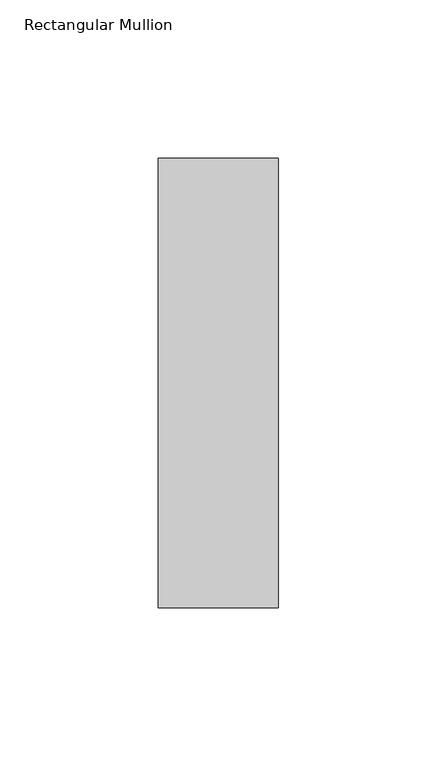
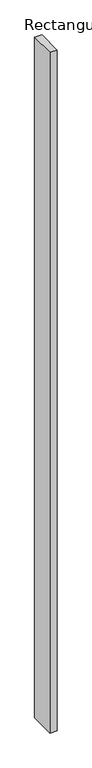
"""IFC4 building model written with IfcOpenShell, lengths in millimetres: member geometry, Rectangular Mullion : NLRS_21_CWM_hsb-regel 38x142_gen_rsf."""

from ifc_helpers import new_model, si_unit, frame, origin, place, context, project, spatial, polyline, outline, extrude, source, transform, mapped, element, save


def rectangular_mullion_f62802ff(model_context):
    return source(origin(), model_context, "Body", "SweptSolid", [
        extrude(outline(polyline([(0.0, -71.0), (-38.0, -71.0), (-38.0, 71.0), (0.0, 71.0), (0.0, -71.0)])), frame((0.0, 0.0, -3849.0), z_axis=(0.0, 0.0, 1.0), x_axis=(1.0, 0.0, 0.0)), (0.0, 0.0, 1.0), 3849.0),
    ])


if __name__ == "__main__":
    model = new_model("IFC4")
    model_context = context("Model", 3, world=origin())
    ifc_project = project(units=[si_unit("LENGTHUNIT", "METRE", prefix="MILLI")], contexts=[model_context])
    site = spatial("IfcSite", under=ifc_project)
    building = spatial("IfcBuilding", under=site)
    placement = place(None, origin())
    rectangular_mullion_shape = rectangular_mullion_f62802ff(model_context)
    element("IfcMember", 1, ObjectType="Rectangular Mullion : NLRS_21_CWM_hsb-regel 38x142_gen_rsf", at=placement, inside=building, context=model_context, shape_type="MappedRepresentation", body=[
        mapped(rectangular_mullion_shape, transform((0.0, 0.0, 0.0), x_axis=(1.0, 0.0, 0.0), y_axis=(0.0, 1.0, 0.0), z_axis=(0.0, 0.0, 1.0))),
    ])
    save(model, "model.ifc")

# Revit data of these elements
# Type "Rectangular Mullion : NLRS_21_CWM_hsb-regel 38x142_gen_rsf"
#   Export Type to IFC As = "IfcWall"
#   Type IfcGUID = "07M7mRoiH1CR8m_RSKIwpF"
#   Assembly Code = "21.10"
#   built-in parameter 1007322 = 0.465879 (stored number, unit not read)
#   built-in parameter 1007321 = 0.062336 (stored number, unit not read)
#   built-in parameter 1007320 = 0.062336 (stored number, unit not read)
# Element 1 (IfcMember, "Rectangular Mullion : NLRS_21_CWM_hsb-regel 38x142_gen_rsf")
#   Materials on its faces: "NLRS_i2_hout naaldhout vuren_gen_rsf"
# Materials
#   "NLRS_i2_hout naaldhout vuren_gen_rsf": class "I - Hout", colour RGB 234 199 147, transparency 0, Keynote = "i2", Manufacturer = "Revit Standards Foundation", URL = "www.revitstandards.org", Description = "hout vuren", Cost = 0
